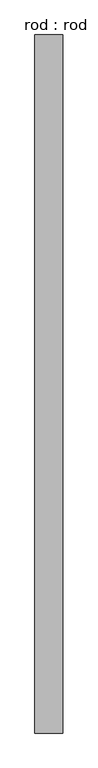
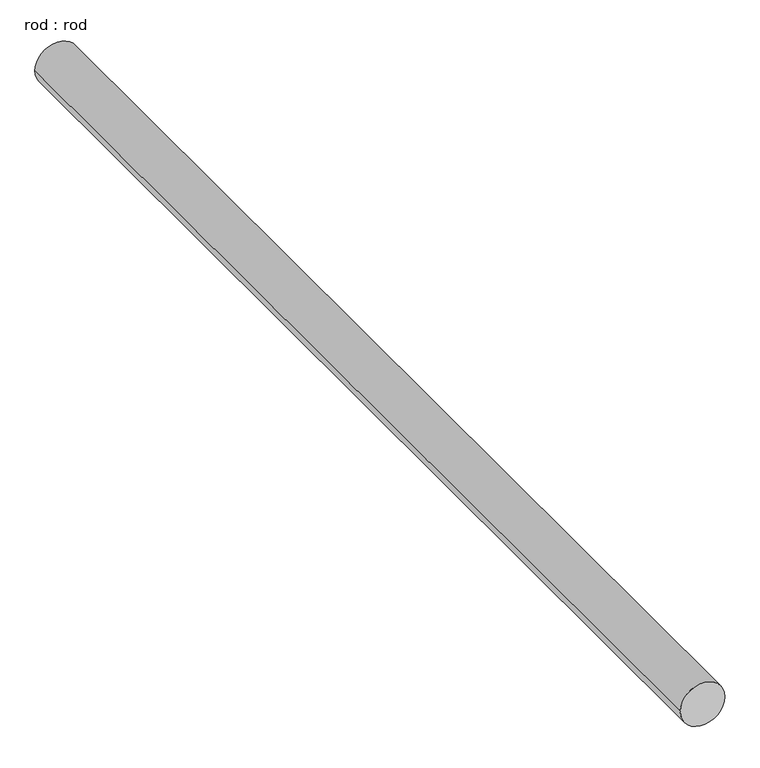
"""IFC4 building model written with IfcOpenShell, lengths in millimetres: proxy geometry, rod : rod."""

from ifc_helpers import new_model, si_unit, point, frame, frame_2d, origin, place, context, project, spatial, circle_curve, trimmed, segment, composite_curve, outline, extrude, source, transform, mapped, element, save


def rod_rod_b4eebbc3(model_context):
    return source(origin(), model_context, "Body", "SweptSolid", [
        extrude(outline(composite_curve([segment(trimmed(circle_curve(frame_2d((0.0108462, 0.0)), 200.0), [point((0.0108462, 200.0))], [point((0.0108462, -200.0))], False, "CARTESIAN"), True, "CONTINUOUS"), segment(trimmed(circle_curve(frame_2d((0.0108462, 0.0)), 200.0), [point((0.0108462, -200.0))], [point((0.0108462, 200.0))], False, "CARTESIAN"), True, "CONTINUOUS")], self_intersect=False)), frame((0.0, -907.2713847, 0.0), z_axis=(0.0, 1.0, 0.0), x_axis=(0.0, 0.0, 1.0)), (0.0, 0.0, 1.0), 10000.0),
    ])


if __name__ == "__main__":
    model = new_model("IFC4")
    model_context = context("Model", 3, world=origin())
    ifc_project = project(units=[si_unit("LENGTHUNIT", "METRE", prefix="MILLI")], contexts=[model_context])
    site = spatial("IfcSite", under=ifc_project)
    building = spatial("IfcBuilding", under=site)
    placement = place(None, origin())
    rod_rod_shape = rod_rod_b4eebbc3(model_context)
    element("IfcBuildingElementProxy", 1, Name="rod : rod", ObjectType="rod : rod", at=placement, inside=building, context=model_context, shape_type="MappedRepresentation", body=[
        mapped(rod_rod_shape, transform((0.0, 0.0, 0.0), x_axis=(1.0, 0.0, 0.0), y_axis=(0.0, 1.0, 0.0), z_axis=(0.0, 0.0, 1.0))),
    ])
    save(model, "model.ifc")

# Revit data of these elements
# Type "rod : rod"
#   Default Elevation = 0
